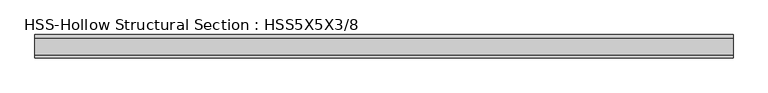
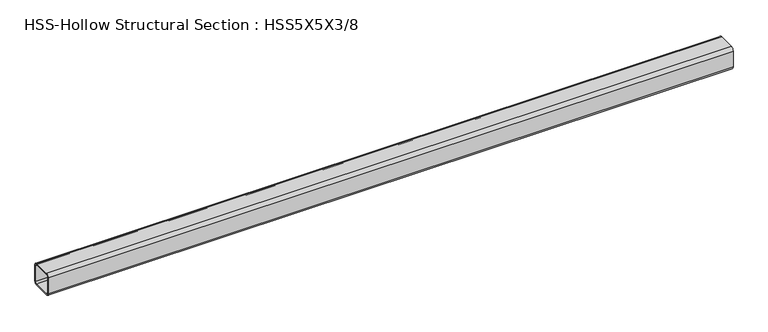
"""IFC4 building model written with IfcOpenShell, lengths in millimetres: member geometry, HSS-Hollow Structural Section : HSS5X5X3/8."""

from ifc_helpers import new_model, si_unit, point, frame, frame_2d, origin, place, context, project, spatial, polyline, circle_curve, trimmed, segment, composite_curve, outline, extrude, source, transform, mapped, element, save


def hss_hollow_structural_section_hss5x5x3_8_86113892(model_context):
    return source(origin(), model_context, "Body", "SweptSolid", [
        extrude(outline(composite_curve([segment(polyline([(63.5, 45.7708), (63.5, -45.7708)]), True, "CONTINUOUS"), segment(trimmed(circle_curve(frame_2d((45.7708, -45.7708)), 17.7292), [point((63.5, -45.7708))], [point((45.7708, -63.5))], False, "CARTESIAN"), True, "CONTINUOUS"), segment(polyline([(45.7708, -63.5), (-45.7708, -63.5)]), True, "CONTINUOUS"), segment(trimmed(circle_curve(frame_2d((-45.7708, -45.7708)), 17.7292), [point((-45.7708, -63.5))], [point((-63.5, -45.7708))], False, "CARTESIAN"), True, "CONTINUOUS"), segment(polyline([(-63.5, -45.7708), (-63.5, 45.7708)]), True, "CONTINUOUS"), segment(trimmed(circle_curve(frame_2d((-45.7708, 45.7708)), 17.7292), [point((-63.5, 45.7708))], [point((-45.7708, 63.5))], False, "CARTESIAN"), True, "CONTINUOUS"), segment(polyline([(-45.7708, 63.5), (45.7708, 63.5)]), True, "CONTINUOUS"), segment(trimmed(circle_curve(frame_2d((45.7708, 45.7708)), 17.7292), [point((45.7708, 63.5))], [point((63.5, 45.7708))], False, "CARTESIAN"), True, "CONTINUOUS")], self_intersect=False), holes=[composite_curve([segment(trimmed(circle_curve(frame_2d((-45.7708, 45.7708)), 8.8646), [point((-45.7708, 54.6354))], [point((-54.6354, 45.7708))], True, "CARTESIAN"), True, "CONTINUOUS"), segment(polyline([(-54.6354, 45.7708), (-54.6354, -45.7708)]), True, "CONTINUOUS"), segment(trimmed(circle_curve(frame_2d((-45.7708, -45.7708)), 8.8646), [point((-54.6354, -45.7708))], [point((-45.7708, -54.6354))], True, "CARTESIAN"), True, "CONTINUOUS"), segment(polyline([(-45.7708, -54.6354), (45.7708, -54.6354)]), True, "CONTINUOUS"), segment(trimmed(circle_curve(frame_2d((45.7708, -45.7708)), 8.8646), [point((45.7708, -54.6354))], [point((54.6354, -45.7708))], True, "CARTESIAN"), True, "CONTINUOUS"), segment(polyline([(54.6354, -45.7708), (54.6354, 45.7708)]), True, "CONTINUOUS"), segment(trimmed(circle_curve(frame_2d((45.7708, 45.7708)), 8.8646), [point((54.6354, 45.7708))], [point((45.7708, 54.6354))], True, "CARTESIAN"), True, "CONTINUOUS"), segment(polyline([(45.7708, 54.6354), (-45.7708, 54.6354)]), True, "CONTINUOUS")], self_intersect=False)]), frame((-1783.4477506, 0.0, 0.0), z_axis=(1.0, 0.0, 0.0), x_axis=(0.0, 1.0, 0.0)), (0.0, 0.0, 1.0), 3778.090058),
    ])


if __name__ == "__main__":
    model = new_model("IFC4")
    model_context = context("Model", 3, world=origin())
    ifc_project = project(units=[si_unit("LENGTHUNIT", "METRE", prefix="MILLI")], contexts=[model_context])
    site = spatial("IfcSite", under=ifc_project)
    building = spatial("IfcBuilding", under=site)
    placement = place(None, origin())
    hss_hollow_structural_section_hss5x5x3_8_shape = hss_hollow_structural_section_hss5x5x3_8_86113892(model_context)
    element("IfcMember", 1, ObjectType="HSS-Hollow Structural Section : HSS5X5X3/8", at=placement, inside=building, context=model_context, shape_type="MappedRepresentation", body=[
        mapped(hss_hollow_structural_section_hss5x5x3_8_shape, transform((0.0, 0.0, 0.0), x_axis=(1.0, 0.0, 0.0), y_axis=(0.0, 1.0, 0.0), z_axis=(0.0, 0.0, 1.0))),
    ])
    save(model, "model.ifc")

# Revit data of these elements
# Type "HSS-Hollow Structural Section : HSS5X5X3/8"
#   Assembly Code = "B10"
#   Shape = "Square"
#   W = 22.3
#   Ht = 0' - 5"
#   Length [instance default] = 5' - 0"
#   b = 0' - 5"
#   kr = 0' - 0.698"
#   t = 0' - 0.349"
#   A = 0.0429167 SF
#   Structural Material [instance default] = Steel ASTM A500, Grade B, Rectangular and Square
# Element 1 (IfcMember, "HSS-Hollow Structural Section : HSS5X5X3/8")
#   Materials on its faces: "Steel ASTM A500, Grade B, Rectangular and Square"
# Materials
#   "Steel ASTM A500, Grade B, Rectangular and Square": class "Metal", colour RGB 199 199 199, transparency 0, Description = "Carbon steel", Cost = 0
